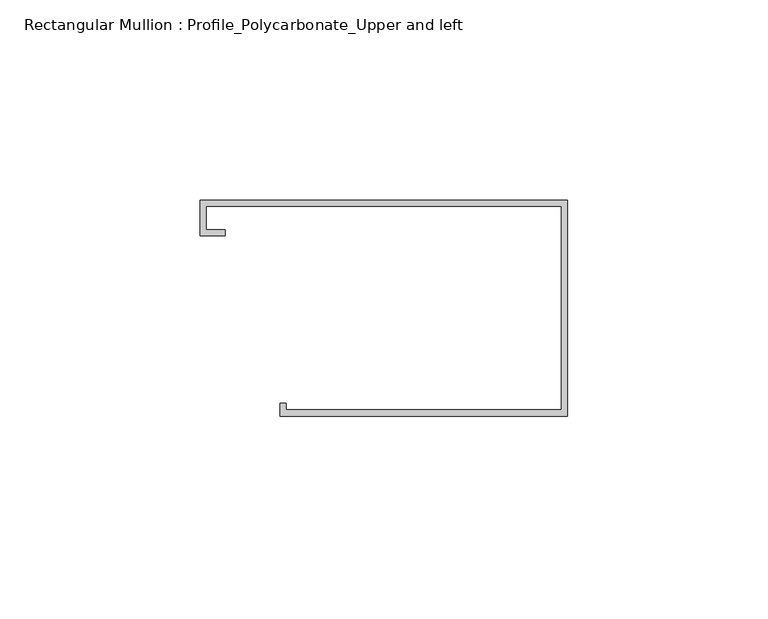
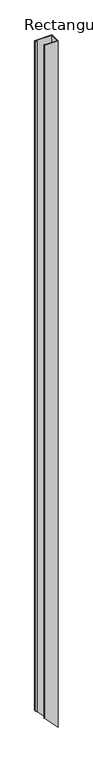
"""IFC4 building model written with IfcOpenShell, lengths in millimetres: member geometry, Rectangular Mullion : Profile_Polycarbonate_Upper and left."""

from ifc_helpers import new_model, si_unit, origin, place, context, project, spatial, faceted_brep, source, transform, mapped, element, save


def rectangular_mullion_profile_polycarbonate_upper_and_left_bead4aea(model_context):
    return source(origin(), model_context, "Body", "Brep", [
        faceted_brep([(0.0, 28.984575, 0.0), (-91.9988, 28.984575, 0.0), (-91.9988, 19.992975, 0.0), (-85.6488, 19.992975, 0.0), (-85.6488, 21.580475, 0.0), (-90.4113, 21.580475, 0.0), (-90.4113, 27.397075, 0.0), (-1.5875, 27.397075, 0.0), (-1.5875, -23.428325, 0.0), (-70.3961, -23.428325, 0.0), (-70.3961, -21.840825, 0.0), (-71.9836, -21.840825, 0.0), (-71.9836, -25.015825, 0.0), (0.0, -25.015825, 0.0), (0.0, 28.984575, -3845.6571133), (-91.9988, 28.984575, -3749.7452045), (-91.9988, 19.992975, -3749.7452045), (-85.6488, 19.992975, -3756.3652976), (-85.6488, 21.580475, -3756.3652976), (-90.4113, 21.580475, -3751.4002278), (-90.4113, 27.397075, -3751.4002278), (-1.5875, 27.397075, -3844.00209), (-1.5875, -23.428325, -3844.00209), (-70.3961, -23.428325, -3772.2667612), (-70.3961, -21.840825, -3772.2667612), (-71.9836, -21.840825, -3770.611738), (-71.9836, -25.015825, -3770.611738), (0.0, -25.015825, -3845.6571133)], [[[0, 1, 2, 3, 4, 5, 6, 7, 8, 9, 10, 11, 12, 13]], [[1, 0, 14, 15]], [[2, 1, 15, 16]], [[3, 2, 16, 17]], [[4, 3, 17, 18]], [[5, 4, 18, 19]], [[6, 5, 19, 20]], [[7, 6, 20, 21]], [[8, 7, 21, 22]], [[9, 8, 22, 23]], [[10, 9, 23, 24]], [[11, 10, 24, 25]], [[12, 11, 25, 26]], [[13, 12, 26, 27]], [[0, 13, 27, 14]], [[14, 27, 26, 25, 24, 23, 22, 21, 20, 19, 18, 17, 16, 15]]]),
    ])


if __name__ == "__main__":
    model = new_model("IFC4")
    model_context = context("Model", 3, world=origin())
    ifc_project = project(units=[si_unit("LENGTHUNIT", "METRE", prefix="MILLI")], contexts=[model_context])
    site = spatial("IfcSite", under=ifc_project)
    building = spatial("IfcBuilding", under=site)
    placement = place(None, origin())
    rectangular_mullion_profile_polycarbonate_upper_and_left_shape = rectangular_mullion_profile_polycarbonate_upper_and_left_bead4aea(model_context)
    element("IfcMember", 1, ObjectType="Rectangular Mullion : Profile_Polycarbonate_Upper and left", at=placement, inside=building, context=model_context, shape_type="MappedRepresentation", body=[
        mapped(rectangular_mullion_profile_polycarbonate_upper_and_left_shape, transform((0.0, 0.0, 0.0), x_axis=(1.0, 0.0, 0.0), y_axis=(0.0, 1.0, 0.0), z_axis=(0.0, 0.0, 1.0))),
    ])
    save(model, "model.ifc")

# Revit data of these elements
# Type "Rectangular Mullion : Profile_Polycarbonate_Upper and left"
#   built-in parameter 1007322 = 0.177167 (stored number, unit not read)
#   built-in parameter 1007321 = 0.00520833 (stored number, unit not read)
#   built-in parameter 1007320 = 0 (stored number, unit not read)
